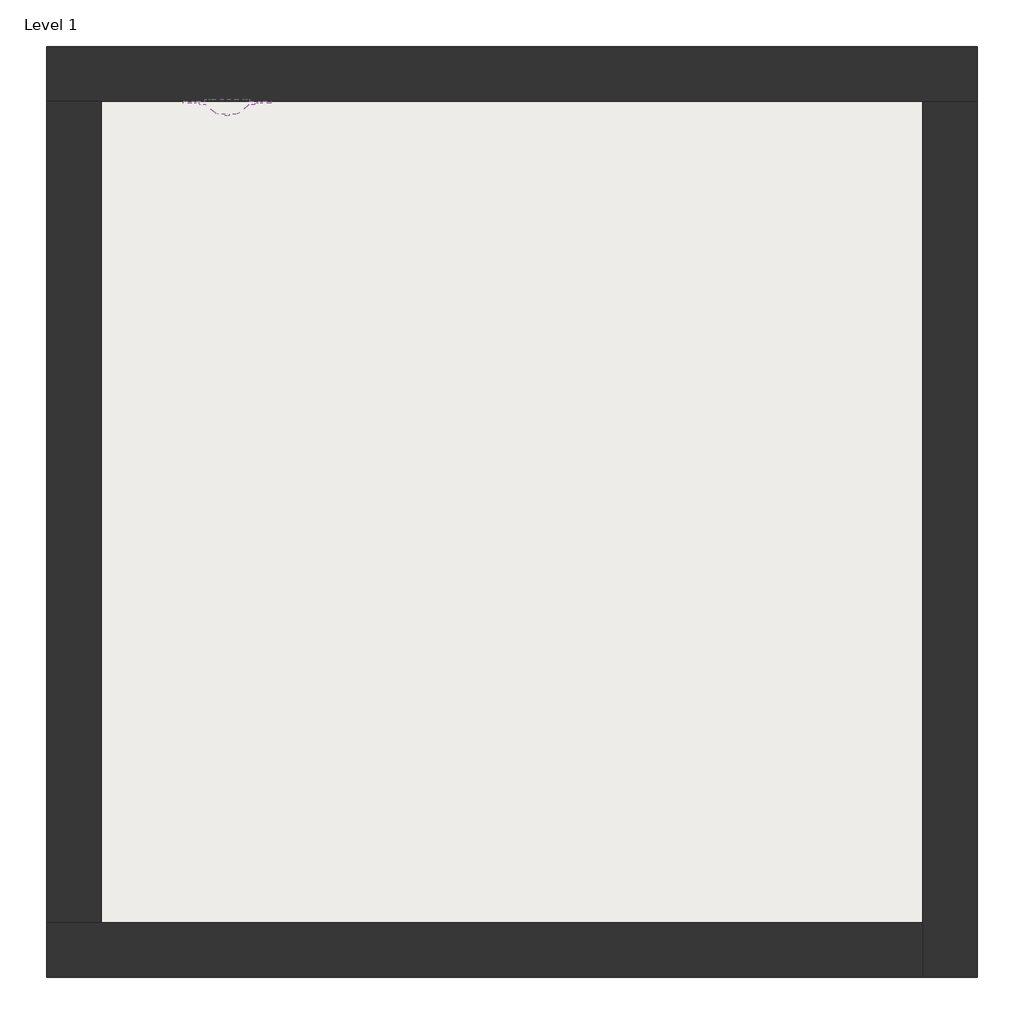
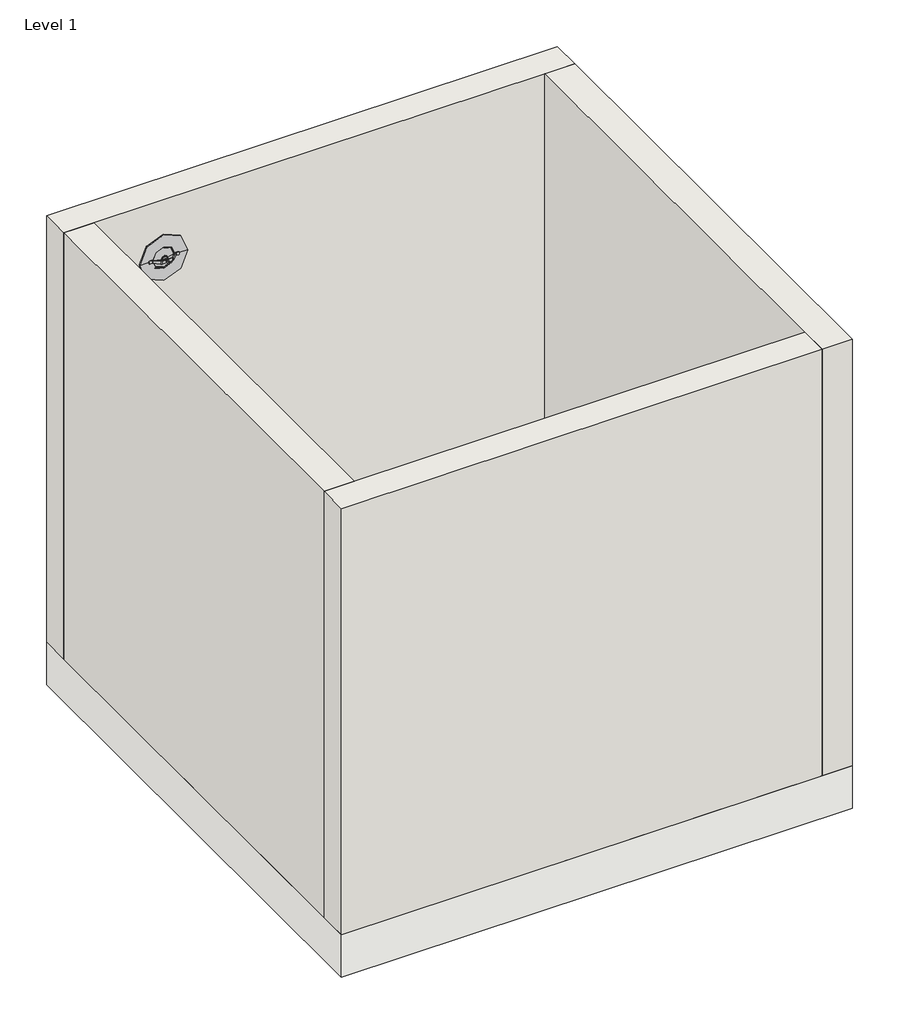
# One storey: 4 walls, 1 proxy, 1 slab.
"""IFC4 building model written with IfcOpenShell, lengths in millimetres."""

import ifcopenshell
import ifcopenshell.guid

model = None  # the IFC model being written
_history = None  # IfcOwnerHistory: only IFC2X3 demands one
_inside = {}  # id of a spatial element -> (the spatial element, [elements in it])
_under = {}  # id of a project, library or spatial element -> (it, [spatial elements below it])
_declared = {}  # id of a project -> (the project, [libraries it declares])
_typed = {}  # id of a type object -> (the type object, [elements of that type])
_made_of = {}  # id of a material, layer set ... -> (it, [elements and type objects made of it])


def new_model(schema):
    """Start an empty IFC model of exactly this schema.

    Asked for "IFC4X3", IfcOpenShell would pick the latest addendum, in which some entities
    have other attributes; the version numbers below select the first issue.
    IFC2X3 requires an IfcOwnerHistory on every rooted entity: one is made here for all.
    """
    global model, _history
    if schema == "IFC4X3":
        model = ifcopenshell.file(schema_version=(4, 3, 0, 0))
    else:
        model = ifcopenshell.file(schema=schema)
    _inside.clear()
    _under.clear()
    _declared.clear()
    _typed.clear()
    _made_of.clear()
    _history = None
    if model.schema == "IFC2X3":
        org = make("IfcOrganization", Name="unknown")
        user = make(
            "IfcPersonAndOrganization",
            ThePerson=make("IfcPerson", FamilyName="unknown"),
            TheOrganization=org,
        )
        app = make(
            "IfcApplication",
            ApplicationDeveloper=org,
            Version="unknown",
            ApplicationFullName="unknown",
            ApplicationIdentifier="unknown",
        )
        _history = make(
            "IfcOwnerHistory",
            OwningUser=user,
            OwningApplication=app,
            ChangeAction="ADDED",
            CreationDate=0,
        )
    return model


def make(cls, **values):
    """One entity of the class cls with the attributes given. An attribute that is None is left unset."""
    return model.create_entity(
        cls, **{name: value for name, value in values.items() if value is not None}
    )


def rooted(cls, **values):
    """An entity with a GlobalId (a new one), such as an element, a storey or a relation."""
    return make(cls, GlobalId=ifcopenshell.guid.new(), OwnerHistory=_history, **values)


def si_unit(unit_type, name, prefix=None):
    """IfcSIUnit, for example si_unit("LENGTHUNIT", "METRE", prefix="MILLI")."""
    return make("IfcSIUnit", UnitType=unit_type, Prefix=prefix, Name=name)


def assignment(units):
    """IfcUnitAssignment: the units of a project."""
    return None if units is None else make("IfcUnitAssignment", Units=units)


def point(xyz):
    """IfcCartesianPoint."""
    return None if xyz is None else make("IfcCartesianPoint", Coordinates=xyz)


def direction(xyz):
    """IfcDirection."""
    return None if xyz is None else make("IfcDirection", DirectionRatios=xyz)


def frame(location, z_axis=None, x_axis=None):
    """IfcAxis2Placement3D, a coordinate frame: its origin and axes. An axis left out is left unset."""
    return make(
        "IfcAxis2Placement3D",
        Location=point(location),
        Axis=direction(z_axis),
        RefDirection=direction(x_axis),
    )


def origin():
    """The frame at (0, 0, 0) with its axes left unset."""
    return frame((0.0, 0.0, 0.0))


def origin_with_axes():
    """The frame at (0, 0, 0) with the z axis (0, 0, 1) and the x axis (1, 0, 0) written out."""
    return frame((0.0, 0.0, 0.0), z_axis=(0.0, 0.0, 1.0), x_axis=(1.0, 0.0, 0.0))


def place(relative_to, where):
    """IfcLocalPlacement: puts the frame where relative to a parent placement (None: the world)."""
    return make(
        "IfcLocalPlacement", PlacementRelTo=relative_to, RelativePlacement=where
    )


def context(
    kind, dimensions, precision=None, world=None, true_north=None, identifier=None
):
    """IfcGeometricRepresentationContext, for example the 3D "Model" context."""
    return make(
        "IfcGeometricRepresentationContext",
        ContextIdentifier=identifier,
        ContextType=kind,
        CoordinateSpaceDimension=dimensions,
        Precision=precision,
        WorldCoordinateSystem=world,
        TrueNorth=true_north,
    )


def project(units=None, contexts=None):
    """IfcProject with its units and contexts."""
    return rooted(
        "IfcProject",
        Name="project",
        RepresentationContexts=contexts,
        UnitsInContext=assignment(units),
    )


def spatial(cls, under=None, at=None, **own):
    """A site, building, storey or space (cls), placed at a placement, below another one or the project."""
    s = rooted(cls, ObjectPlacement=at, **own)
    if under is not None:
        _under.setdefault(under.id(), (under, []))[1].append(s)
    return s


def polyline(points):
    """IfcPolyline through the points."""
    return make("IfcPolyline", Points=[point(p) for p in points])


def circle_curve(where, radius):
    """IfcCircle in the frame where."""
    return make("IfcCircle", Position=where, Radius=radius)


def ellipse_curve(where, semi_axis1, semi_axis2):
    """IfcEllipse in the frame where."""
    return make(
        "IfcEllipse", Position=where, SemiAxis1=semi_axis1, SemiAxis2=semi_axis2
    )


def trimmed(basis, trim1, trim2, sense, master):
    """IfcTrimmedCurve: the piece of a basis curve between two trims."""
    return make(
        "IfcTrimmedCurve",
        BasisCurve=basis,
        Trim1=trim1,
        Trim2=trim2,
        SenseAgreement=sense,
        MasterRepresentation=master,
    )


def outline(outer, holes=None, kind="AREA"):
    """IfcArbitraryClosedProfileDef: a profile drawn as a closed curve; with holes, ...WithVoids."""
    if holes is None:
        return make("IfcArbitraryClosedProfileDef", ProfileType=kind, OuterCurve=outer)
    return make(
        "IfcArbitraryProfileDefWithVoids",
        ProfileType=kind,
        OuterCurve=outer,
        InnerCurves=holes,
    )


def extrude(swept, where, along, depth):
    """IfcExtrudedAreaSolid: the profile swept, set in the frame where, extruded along a direction by depth."""
    return make(
        "IfcExtrudedAreaSolid",
        SweptArea=swept,
        Position=where,
        ExtrudedDirection=direction(along),
        Depth=depth,
    )


def faces_of(points, faces, orient=None, outer=None):
    """IfcFace entities. A face is a list of loops; a loop is a list of indices into points, from 0.

    orient and outer hold one flag for each loop. By default every Orientation is true, the
    first loop of a face is its IfcFaceOuterBound and the others are IfcFaceBound.
    """
    made = []
    for i, loops in enumerate(faces):
        bounds = []
        for j, loop in enumerate(loops):
            is_outer = j == 0 if outer is None else outer[i][j]
            bounds.append(
                make(
                    "IfcFaceOuterBound" if is_outer else "IfcFaceBound",
                    Bound=make("IfcPolyLoop", Polygon=[points[k] for k in loop]),
                    Orientation=True if orient is None else orient[i][j],
                )
            )
        made.append(make("IfcFace", Bounds=bounds))
    return made


def faceted_brep(points, faces, orient=None, outer=None, voids=None):
    """IfcFacetedBrep: a solid bounded by flat faces; with voids (closed shells), ...WithVoids."""
    shared = [point(p) for p in points]
    hull = make("IfcClosedShell", CfsFaces=faces_of(shared, faces, orient, outer))
    if voids is None:
        return make("IfcFacetedBrep", Outer=hull)
    return make(
        "IfcFacetedBrepWithVoids",
        Outer=hull,
        Voids=[
            make(cls, CfsFaces=faces_of(shared, fs, o, b)) for cls, fs, o, b in voids
        ],
    )


def shape(context_of_items, identifier, shape_type, items):
    """IfcShapeRepresentation: the items that make up one representation, for example the "Body"."""
    return make(
        "IfcShapeRepresentation",
        ContextOfItems=context_of_items,
        RepresentationIdentifier=identifier,
        RepresentationType=shape_type,
        Items=items,
    )


def source(mapping_origin, context_of_items, identifier, shape_type, items):
    """IfcRepresentationMap: a shape defined once, which mapped items show again and again."""
    return make(
        "IfcRepresentationMap",
        MappingOrigin=mapping_origin,
        MappedRepresentation=shape(context_of_items, identifier, shape_type, items),
    )


def transform(
    local_origin,
    x_axis=None,
    y_axis=None,
    z_axis=None,
    scale=None,
    scale2=None,
    scale3=None,
    uniform=True,
):
    """IfcCartesianTransformationOperator3D, or its non-uniform kind. x_axis, y_axis, z_axis: its Axis1, 2, 3."""
    if uniform:
        return make(
            "IfcCartesianTransformationOperator3D",
            Axis1=direction(x_axis),
            Axis2=direction(y_axis),
            LocalOrigin=point(local_origin),
            Scale=scale,
            Axis3=direction(z_axis),
        )
    return make(
        "IfcCartesianTransformationOperator3DnonUniform",
        Axis1=direction(x_axis),
        Axis2=direction(y_axis),
        LocalOrigin=point(local_origin),
        Scale=scale,
        Axis3=direction(z_axis),
        Scale2=scale2,
        Scale3=scale3,
    )


def mapped(mapping_source, mapping_target):
    """IfcMappedItem: shows the shape of a source again, moved by a transform."""
    return make(
        "IfcMappedItem", MappingSource=mapping_source, MappingTarget=mapping_target
    )


def made_of(thing, what):
    """Note that an element or type object is made of a material, layer set ...; save() writes the relation."""
    if what is not None:
        _made_of.setdefault(what.id(), (what, []))[1].append(thing)
    return thing


def element(
    cls,
    number,
    at=None,
    inside=None,
    cuts=None,
    type_object=None,
    material=None,
    context=None,
    identifier="Body",
    shape_type=None,
    held_by="IfcProductDefinitionShape",
    body=None,
    shapes=None,
    **own,
):
    """One element of the class cls, such as IfcWall. Its Tag is "e" and its number.

    at: its placement. inside: the storey or other place that contains it. cuts: it is an
    opening in that element (IfcRelVoidsElement). A single representation is given by context,
    identifier, shape_type and body (its items); several are given by shapes. held_by: the class
    of the entity that holds the representations. save() writes the other relations.
    """
    e = rooted(cls, Tag="e%d" % number, ObjectPlacement=at, **own)
    if body is not None:
        shapes = [shape(context, identifier, shape_type, body)]
    if shapes is not None:
        e.Representation = make(held_by, Representations=shapes)
    if inside is not None:
        _inside.setdefault(inside.id(), (inside, []))[1].append(e)
    if cuts is not None:
        rooted(
            "IfcRelVoidsElement", RelatingBuildingElement=cuts, RelatedOpeningElement=e
        )
    if type_object is not None:
        _typed.setdefault(type_object.id(), (type_object, []))[1].append(e)
    return made_of(e, material)


def aggregate(whole, parts):
    """IfcRelAggregates: a whole, such as a stair, and the parts it consists of."""
    return rooted("IfcRelAggregates", RelatingObject=whole, RelatedObjects=parts)


def save(model, path):
    """Write the relations noted so far, then the file.

    IfcRelAggregates (storeys below a building ...), IfcRelContainedInSpatialStructure (elements
    in a storey), IfcRelDefinesByType, IfcRelAssociatesMaterial and IfcRelDeclares: one each for
    every whole, place, type object, material and project.
    """
    for whole, parts in _under.values():
        aggregate(whole, parts)
    for where, things in _inside.values():
        rooted(
            "IfcRelContainedInSpatialStructure",
            RelatedElements=things,
            RelatingStructure=where,
        )
    for kind, things in _typed.values():
        rooted("IfcRelDefinesByType", RelatedObjects=things, RelatingType=kind)
    for what, things in _made_of.values():
        rooted("IfcRelAssociatesMaterial", RelatedObjects=things, RelatingMaterial=what)
    for by, libraries in _declared.values():
        rooted("IfcRelDeclares", RelatingContext=by, RelatedDefinitions=libraries)
    model.write(path)


def plane_surface(at):
    """IfcPlane: the flat surface through the origin of the frame at, square to its z axis."""
    return make("IfcPlane", Position=at)


def cylinder_surface(at, radius):
    """IfcCylindricalSurface: all points at the distance radius from the z axis of the frame at."""
    return make("IfcCylindricalSurface", Position=at, Radius=radius)


def revolved_surface(curve, axis_point, axis_direction):
    """IfcSurfaceOfRevolution: the curve turned about the line through axis_point along axis_direction."""
    return make(
        "IfcSurfaceOfRevolution",
        SweptCurve=make("IfcArbitraryOpenProfileDef", ProfileType="CURVE", Curve=curve),
        AxisPosition=make("IfcAxis1Placement", Location=point(axis_point), Axis=direction(axis_direction)),
    )


def advanced_brep(points, edges, surfaces, faces):
    """IfcAdvancedBrep: a solid bounded by faces that lie on surfaces and meet in shared edges.

    An edge is (start, end): straight between two places in points (the first is 0);
    or (start, end, curve); or (start, end, curve, False) where it runs against its curve.
    A face is (place in surfaces, loops), or (place, loops, False) where it looks against
    its surface's normal. A loop lists edges by number (the first is 1), with a minus sign
    where the edge is run from its end to its start. The first loop is the outer one.
    """
    corners = [point(p) for p in points]
    vertices = [make("IfcVertexPoint", VertexGeometry=c) for c in corners]
    made = []
    for start, end, *more in edges:
        made.append(
            make(
                "IfcEdgeCurve",
                EdgeStart=vertices[start],
                EdgeEnd=vertices[end],
                EdgeGeometry=more[0] if more else make("IfcPolyline", Points=[corners[start], corners[end]]),
                SameSense=more[1] if len(more) > 1 else True,
            )
        )
    hull = []
    for where, loops, *sense in faces:
        bounds = []
        for j, loop in enumerate(loops):
            ring = [make("IfcOrientedEdge", EdgeElement=made[abs(k) - 1], Orientation=k > 0) for k in loop]
            bounds.append(
                make(
                    "IfcFaceOuterBound" if j == 0 else "IfcFaceBound",
                    Bound=make("IfcEdgeLoop", EdgeList=ring),
                    Orientation=True,
                )
            )
        hull.append(make("IfcAdvancedFace", Bounds=bounds, FaceSurface=surfaces[where], SameSense=sense[0] if sense else True))
    return make("IfcAdvancedBrep", Outer=make("IfcClosedShell", CfsFaces=hull))


def mechanical_equipment_492a67d3(model_context):
    return source(origin(), model_context, "Body", "AdvancedBrep", [
        advanced_brep(
        [(44.3795006, 108.0, 2610.0), (54.2298211, 113.0, 2610.0), (87.44309, 140.8692417, 2610.0), (91.8102497, 143.0, 2610.0), (125.0, 143.0, 2610.0), (158.1897503, 143.0, 2610.0), (162.55691, 140.8692417, 2610.0), (195.7701789, 113.0, 2610.0), (205.6204994, 108.0, 2610.0), (221.2200072, 108.0, 2610.0), (221.2200072, 113.0, 2610.0), (205.6204994, 113.0, 2610.0), (201.5540671, 114.8851429, 2610.0), (165.874925, 144.8234979, 2610.0), (158.1897503, 148.0, 2610.0), (125.0, 148.0, 2610.0), (91.8102497, 148.0, 2610.0), (84.125075, 144.8234979, 2610.0), (48.4459329, 114.8851429, 2610.0), (44.3795006, 113.0, 2610.0), (28.7799928, 113.0, 2610.0), (28.7799928, 108.0, 2610.0), (44.3795006, 113.0, 2590.0), (48.4459329, 114.8851429, 2590.0), (84.125075, 144.8234979, 2590.0), (91.8102497, 148.0, 2590.0), (125.0, 148.0, 2590.0), (158.1897503, 148.0, 2590.0), (165.874925, 144.8234979, 2590.0), (201.5540671, 114.8851429, 2590.0), (205.6204994, 113.0, 2590.0), (221.2200072, 113.0, 2590.0), (221.2200072, 108.0, 2590.0), (205.6204994, 108.0, 2590.0), (195.7701789, 113.0, 2590.0), (162.55691, 140.8692417, 2590.0), (158.1897503, 143.0, 2590.0), (125.0, 143.0, 2590.0), (91.8102497, 143.0, 2590.0), (87.44309, 140.8692417, 2590.0), (54.2298211, 113.0, 2590.0), (44.3795006, 108.0, 2590.0), (28.7799928, 108.0, 2590.0), (28.7799928, 113.0, 2590.0), (25.0, 108.0, 2606.2200072), (25.0, 108.0, 2593.7799928), (225.0, 108.0, 2593.7799928), (225.0, 108.0, 2606.2200072), (225.0, 113.0, 2593.7799928), (225.0, 113.0, 2606.2200072), (25.0, 113.0, 2593.7799928), (25.0, 113.0, 2606.2200072)],
        [
            (0, 1, circle_curve(frame((38.5511411, 131.6851233, 2610.0), z_axis=(0.0, 0.0, 1.0), x_axis=(1.0, 0.0, 0.0)), 24.3916961)),
            (1, 2),
            (2, 3, circle_curve(frame((93.9022065, 133.1715663, 2610.0), z_axis=(0.0, 0.0, -1.0), x_axis=(1.0, 0.0, 0.0)), 10.0486015)),
            (3, 4),
            (4, 5),
            (5, 6, circle_curve(frame((156.0977935, 133.1715663, 2610.0), z_axis=(0.0, 0.0, -1.0), x_axis=(-1.0, 0.0, 0.0)), 10.0486015)),
            (6, 7),
            (7, 8, circle_curve(frame((211.4488589, 131.6851233, 2610.0), z_axis=(0.0, 0.0, 1.0), x_axis=(-1.0, 0.0, 0.0)), 24.3916961)),
            (8, 9),
            (9, 10),
            (10, 11),
            (11, 12, circle_curve(frame((205.6204994, 118.3284116, 2610.0), z_axis=(0.0, 0.0, -1.0), x_axis=(-1.0, 0.0, 0.0)), 5.3284116)),
            (12, 13),
            (13, 14, circle_curve(frame((158.1897503, 137.115059, 2610.0), z_axis=(0.0, 0.0, 1.0), x_axis=(-1.0, 0.0, 0.0)), 10.884941)),
            (14, 15),
            (15, 16),
            (16, 17, circle_curve(frame((91.8102497, 137.115059, 2610.0), z_axis=(0.0, 0.0, 1.0), x_axis=(1.0, 0.0, 0.0)), 10.884941)),
            (17, 18),
            (18, 19, circle_curve(frame((44.3795006, 118.3284116, 2610.0), z_axis=(0.0, 0.0, -1.0), x_axis=(1.0, 0.0, 0.0)), 5.3284116)),
            (19, 20),
            (20, 21),
            (21, 0),
            (22, 23, circle_curve(frame((44.3795006, 118.3284116, 2590.0), z_axis=(0.0, 0.0, 1.0), x_axis=(1.0, 0.0, 0.0)), 5.3284116)),
            (23, 24),
            (24, 25, circle_curve(frame((91.8102497, 137.115059, 2590.0), z_axis=(0.0, 0.0, -1.0), x_axis=(1.0, 0.0, 0.0)), 10.884941)),
            (25, 26),
            (26, 27),
            (27, 28, circle_curve(frame((158.1897503, 137.115059, 2590.0), z_axis=(0.0, 0.0, -1.0), x_axis=(-1.0, 0.0, 0.0)), 10.884941)),
            (28, 29),
            (29, 30, circle_curve(frame((205.6204994, 118.3284116, 2590.0), z_axis=(0.0, 0.0, 1.0), x_axis=(-1.0, 0.0, 0.0)), 5.3284116)),
            (30, 31),
            (31, 32),
            (32, 33),
            (33, 34, circle_curve(frame((211.4488589, 131.6851233, 2590.0), z_axis=(0.0, 0.0, -1.0), x_axis=(-1.0, 0.0, 0.0)), 24.3916961)),
            (34, 35),
            (35, 36, circle_curve(frame((156.0977935, 133.1715663, 2590.0), z_axis=(0.0, 0.0, 1.0), x_axis=(-1.0, 0.0, 0.0)), 10.0486015)),
            (36, 37),
            (37, 38),
            (38, 39, circle_curve(frame((93.9022065, 133.1715663, 2590.0), z_axis=(0.0, 0.0, 1.0), x_axis=(1.0, 0.0, 0.0)), 10.0486015)),
            (39, 40),
            (40, 41, circle_curve(frame((38.5511411, 131.6851233, 2590.0), z_axis=(0.0, 0.0, -1.0), x_axis=(1.0, 0.0, 0.0)), 24.3916961)),
            (41, 42),
            (42, 43),
            (43, 22),
            (41, 0),
            (21, 44, circle_curve(frame((28.7799928, 108.0, 2606.2200072), z_axis=(0.0, -1.0, 0.0), x_axis=(1.0, 0.0, 0.0)), 3.7799928)),
            (44, 45),
            (45, 42, circle_curve(frame((28.7799928, 108.0, 2593.7799928), z_axis=(0.0, -1.0, 0.0), x_axis=(1.0, 0.0, 0.0)), 3.7799928)),
            (40, 1),
            (39, 2),
            (38, 3),
            (37, 4),
            (36, 5),
            (35, 6),
            (34, 7),
            (33, 8),
            (32, 46, circle_curve(frame((221.2200072, 108.0, 2593.7799928), z_axis=(0.0, -1.0, 0.0), x_axis=(-1.0, 0.0, 0.0)), 3.7799928)),
            (46, 47),
            (47, 9, circle_curve(frame((221.2200072, 108.0, 2606.2200072), z_axis=(0.0, -1.0, 0.0), x_axis=(-1.0, 0.0, 0.0)), 3.7799928)),
            (46, 48),
            (48, 49),
            (49, 47),
            (30, 11),
            (10, 49, circle_curve(frame((221.2200072, 113.0, 2606.2200072), z_axis=(0.0, 1.0, 0.0), x_axis=(-1.0, 0.0, 0.0)), 3.7799928)),
            (48, 31, circle_curve(frame((221.2200072, 113.0, 2593.7799928), z_axis=(0.0, 1.0, 0.0), x_axis=(-1.0, 0.0, 0.0)), 3.7799928)),
            (29, 12),
            (28, 13),
            (27, 14),
            (26, 15),
            (25, 16),
            (24, 17),
            (23, 18),
            (22, 19),
            (43, 50, circle_curve(frame((28.7799928, 113.0, 2593.7799928), z_axis=(0.0, 1.0, 0.0), x_axis=(1.0, 0.0, 0.0)), 3.7799928)),
            (50, 51),
            (51, 20, circle_curve(frame((28.7799928, 113.0, 2606.2200072), z_axis=(0.0, 1.0, 0.0), x_axis=(1.0, 0.0, 0.0)), 3.7799928)),
            (44, 51),
            (50, 45),
        ],
        [
            plane_surface(frame((25.0, 108.0, 2610.0), z_axis=(0.0, 0.0, 1.0), x_axis=(1.0, 0.0, 0.0))),
            plane_surface(frame((25.0, 108.0, 2590.0), z_axis=(0.0, 0.0, -1.0), x_axis=(-1.0, 0.0, 0.0))),
            plane_surface(frame((25.0, 108.0, 2610.0), z_axis=(0.0, -1.0, 0.0), x_axis=(0.0, 0.0, -1.0))),
            cylinder_surface(frame((38.5511411, 131.6851233, 2590.0), z_axis=(0.0, 0.0, 1.0), x_axis=(1.0, 0.0, 0.0)), 24.3916961),
            plane_surface(frame((54.2298211, 113.0, 2610.0), z_axis=(0.6427876096865391, -0.7660444431189783, 0.0), x_axis=(0.0, 0.0, -1.0))),
            revolved_surface(polyline([(103.95080800000001, 133.1715663, 2590.0), (103.95080800000001, 133.1715663, 2610.0)]), (93.9022065, 133.1715663, 2590.0), (0.0, 0.0, -1.0)),
            plane_surface(frame((91.8102497, 143.0, 2610.0), z_axis=(0.0, -1.0, 0.0), x_axis=(0.0, 0.0, -1.0))),
            plane_surface(frame((125.0, 143.0, 2610.0), z_axis=(0.0, -1.0, 0.0), x_axis=(0.0, 0.0, -1.0))),
            revolved_surface(polyline([(146.049192, 133.1715663, 2590.0), (146.049192, 133.1715663, 2610.0)]), (156.0977935, 133.1715663, 2590.0), (0.0, 0.0, -1.0)),
            plane_surface(frame((162.55691, 140.8692417, 2610.0), z_axis=(-0.6427876096865387, -0.7660444431189786, 0.0), x_axis=(0.0, 0.0, -1.0))),
            cylinder_surface(frame((211.4488589, 131.6851233, 2590.0), z_axis=(0.0, 0.0, 1.0), x_axis=(-1.0, 0.0, 0.0)), 24.3916961),
            plane_surface(frame((205.6204994, 108.0, 2610.0), z_axis=(0.0, -1.0, 0.0), x_axis=(0.0, 0.0, -1.0))),
            plane_surface(frame((225.0, 108.0, 2610.0), z_axis=(1.0, 0.0, 0.0), x_axis=(0.0, 0.0, -1.0))),
            plane_surface(frame((225.0, 113.0, 2610.0), z_axis=(0.0, 1.0, 0.0), x_axis=(0.0, 0.0, -1.0))),
            revolved_surface(polyline([(200.2920878, 118.3284116, 2590.0), (200.2920878, 118.3284116, 2610.0)]), (205.6204994, 118.3284116, 2590.0), (0.0, 0.0, -1.0)),
            plane_surface(frame((201.5540671, 114.8851429, 2610.0), z_axis=(0.6427876096865414, 0.7660444431189763, 0.0), x_axis=(0.0, 0.0, -1.0))),
            cylinder_surface(frame((158.1897503, 137.115059, 2590.0), z_axis=(0.0, 0.0, 1.0), x_axis=(-1.0, 0.0, 0.0)), 10.884941),
            plane_surface(frame((158.1897503, 148.0, 2610.0), z_axis=(0.0, 1.0, 0.0), x_axis=(0.0, 0.0, -1.0))),
            plane_surface(frame((125.0, 148.0, 2610.0), z_axis=(0.0, 1.0, 0.0), x_axis=(0.0, 0.0, -1.0))),
            cylinder_surface(frame((91.8102497, 137.115059, 2590.0), z_axis=(0.0, 0.0, 1.0), x_axis=(1.0, 0.0, 0.0)), 10.884941),
            plane_surface(frame((84.125075, 144.8234979, 2610.0), z_axis=(-0.6427876096865359, 0.766044443118981, 0.0), x_axis=(0.0, 0.0, -1.0))),
            revolved_surface(polyline([(49.7079122, 118.3284116, 2590.0), (49.7079122, 118.3284116, 2610.0)]), (44.3795006, 118.3284116, 2590.0), (0.0, 0.0, -1.0)),
            plane_surface(frame((44.3795006, 113.0, 2610.0), z_axis=(0.0, 1.0, 0.0), x_axis=(0.0, 0.0, -1.0))),
            plane_surface(frame((25.0, 113.0, 2610.0), z_axis=(-1.0, 0.0, 0.0), x_axis=(0.0, 0.0, -1.0))),
            cylinder_surface(frame((28.7799928, 108.0, 2593.7799928), z_axis=(0.0, -1.0, 0.0), x_axis=(1.0, 0.0, 0.0)), 3.7799928),
            cylinder_surface(frame((28.7799928, 93.5, 2606.2200072), z_axis=(0.0, -1.0, 0.0), x_axis=(1.0, 0.0, 0.0)), 3.7799928),
            cylinder_surface(frame((221.2200072, 93.5, 2593.7799928), z_axis=(0.0, -1.0, 0.0), x_axis=(-1.0, 0.0, 0.0)), 3.7799928),
            cylinder_surface(frame((221.2200072, 93.5, 2606.2200072), z_axis=(0.0, -1.0, 0.0), x_axis=(-1.0, 0.0, 0.0)), 3.7799928),
        ],
        [
            (0, [[1, 2, 3, 4, 5, 6, 7, 8, 9, 10, 11, 12, 13, 14, 15, 16, 17, 18, 19, 20, 21, 22]]),
            (1, [[23, 24, 25, 26, 27, 28, 29, 30, 31, 32, 33, 34, 35, 36, 37, 38, 39, 40, 41, 42, 43, 44]]),
            (2, [[45, -22, 46, 47, 48, -42]]),
            (3, [[-1, -45, -41, 49]]),
            (4, [[-2, -49, -40, 50]]),
            (5, [[-3, -50, -39, 51]]),
            (6, [[-4, -51, -38, 52]]),
            (7, [[-5, -52, -37, 53]]),
            (8, [[-6, -53, -36, 54]]),
            (9, [[-7, -54, -35, 55]]),
            (10, [[-8, -55, -34, 56]]),
            (11, [[-56, -33, 57, 58, 59, -9]]),
            (12, [[-58, 60, 61, 62]]),
            (13, [[63, -11, 64, -61, 65, -31]]),
            (14, [[-12, -63, -30, 66]]),
            (15, [[-13, -66, -29, 67]]),
            (16, [[-14, -67, -28, 68]]),
            (17, [[-15, -68, -27, 69]]),
            (18, [[-16, -69, -26, 70]]),
            (19, [[-17, -70, -25, 71]]),
            (20, [[-18, -71, -24, 72]]),
            (21, [[-19, -72, -23, 73]]),
            (22, [[-73, -44, 74, 75, 76, -20]]),
            (23, [[-47, 77, -75, 78]]),
            (24, [[-43, -48, -78, -74]]),
            (25, [[-21, -76, -77, -46]]),
            (26, [[-32, -65, -60, -57]]),
            (27, [[-10, -59, -62, -64]]),
        ],
    ),
        advanced_brep(
        [(207.7271571, 93.5, 2600.0), (42.2728429, 93.5, 2600.0), (42.2728429, 97.7728429, 2600.0), (207.7271571, 97.7728429, 2600.0), (205.9367462, 93.5, 2600.0), (44.0632538, 93.5, 2600.0), (205.9367462, 97.9071057, 2600.0), (44.0632538, 97.9071057, 2600.0), (205.3438519, 98.5, 2600.0), (44.6561481, 98.5, 2600.0), (197.7785514, 98.5, 2600.0), (52.2214486, 98.5, 2600.0), (194.5390342, 101.1233093, 2600.0), (55.4609658, 101.1233093, 2600.0), (194.110594, 101.9290881, 2600.0), (55.889406, 101.9290881, 2600.0), (143.1174907, 117.056758, 2600.0), (106.8825093, 117.056758, 2600.0), (139.9690463, 120.2052024, 2600.0), (110.0309537, 120.2052024, 2600.0), (139.3942487, 120.78, 2600.0), (110.6057513, 120.78, 2600.0), (125.0, 120.78, 2600.0), (139.6388233, 122.2731901, 2600.0), (110.3611767, 122.2731901, 2600.0), (120.9566338, 122.2731901, 2600.0), (129.0433662, 122.2731901, 2600.0), (141.5029828, 120.4090307, 2600.0), (108.4970172, 120.4090307, 2600.0), (143.1991524, 118.522856, 2600.0), (106.8008476, 118.522856, 2600.0), (145.9642188, 118.2410596, 2600.0), (104.0357812, 118.2410596, 2600.0), (194.877574, 103.206216, 2600.0), (55.122426, 103.206216, 2600.0), (196.1038029, 101.6367146, 2600.0), (53.8961971, 101.6367146, 2600.0), (198.0543634, 100.0, 2600.0), (51.9456366, 100.0, 2600.0), (200.0, 100.0, 2600.0), (50.0, 100.0, 2600.0), (200.0, 108.0, 2600.0), (50.0, 108.0, 2600.0), (285.0, 108.0, 2600.0), (-35.0, 108.0, 2600.0), (285.0, 100.0, 2600.0), (-35.0, 100.0, 2600.0), (205.5, 100.0, 2600.0), (44.5, 100.0, 2600.0), (133.0867323, 136.6576943, 2600.0), (116.9132677, 136.6576943, 2600.0), (116.9132677, 153.9, 2600.0), (133.0867323, 153.9, 2600.0), (129.0433662, 136.6576943, 2600.0), (120.9566338, 136.6576943, 2600.0), (125.0, 153.9, 2600.0)],
        [
            (0, 1, circle_curve(frame((125.0, 93.5, 2600.0), z_axis=(0.0, 1.0, 0.0), x_axis=(-1.0, 0.0, 0.0)), 82.7271571)),
            (1, 2),
            (2, 3, circle_curve(frame((125.0, 97.7728429, 2600.0), z_axis=(0.0, -1.0, 0.0), x_axis=(-1.0, 0.0, 0.0)), 82.7271571)),
            (3, 0),
            (1, 0, circle_curve(frame((125.0, 93.5, 2600.0), z_axis=(0.0, 1.0, 0.0), x_axis=(-1.0, 0.0, 0.0)), 82.7271571)),
            (3, 2, circle_curve(frame((125.0, 97.7728429, 2600.0), z_axis=(0.0, -1.0, 0.0), x_axis=(-1.0, 0.0, 0.0)), 82.7271571)),
            (0, 4),
            (4, 5, circle_curve(frame((125.0, 93.5, 2600.0), z_axis=(0.0, 1.0, 0.0), x_axis=(-1.0, 0.0, 0.0)), 80.9367462)),
            (5, 1),
            (5, 4, circle_curve(frame((125.0, 93.5, 2600.0), z_axis=(0.0, 1.0, 0.0), x_axis=(-1.0, 0.0, 0.0)), 80.9367462)),
            (4, 6),
            (6, 7, circle_curve(frame((125.0, 97.9071057, 2600.0), z_axis=(0.0, 1.0, 0.0), x_axis=(-1.0, 0.0, 0.0)), 80.9367462)),
            (7, 5),
            (7, 6, circle_curve(frame((125.0, 97.9071057, 2600.0), z_axis=(0.0, 1.0, 0.0), x_axis=(-1.0, 0.0, 0.0)), 80.9367462)),
            (6, 8, circle_curve(frame((205.3438519, 97.9071057, 2600.0), z_axis=(0.0, 0.0, 1.0), x_axis=(-1.0, 0.0, 0.0)), 0.5928943)),
            (8, 9, circle_curve(frame((125.0, 98.5, 2600.0), z_axis=(0.0, 1.0, 0.0), x_axis=(-1.0, 0.0, 0.0)), 80.3438519)),
            (9, 7, circle_curve(frame((44.6561481, 97.9071057, 2600.0), z_axis=(0.0, 0.0, 1.0), x_axis=(1.0, 0.0, 0.0)), 0.5928943)),
            (9, 8, circle_curve(frame((125.0, 98.5, 2600.0), z_axis=(0.0, 1.0, 0.0), x_axis=(-1.0, 0.0, 0.0)), 80.3438519)),
            (8, 10),
            (10, 11, circle_curve(frame((125.0, 98.5, 2600.0), z_axis=(0.0, 1.0, 0.0), x_axis=(-1.0, 0.0, 0.0)), 72.7785514)),
            (11, 9),
            (11, 10, circle_curve(frame((125.0, 98.5, 2600.0), z_axis=(0.0, 1.0, 0.0), x_axis=(-1.0, 0.0, 0.0)), 72.7785514)),
            (10, 12, circle_curve(frame((197.9467336, 102.0195777, 2600.0), z_axis=(0.0, 0.0, -1.0), x_axis=(-1.0, 0.0, 0.0)), 3.5235937)),
            (12, 13, circle_curve(frame((125.0, 101.1233093, 2600.0), z_axis=(0.0, 1.0, 0.0), x_axis=(-1.0, 0.0, 0.0)), 69.5390342)),
            (13, 11, circle_curve(frame((52.0532664, 102.0195777, 2600.0), z_axis=(0.0, 0.0, -1.0), x_axis=(1.0, 0.0, 0.0)), 3.5235937)),
            (13, 12, circle_curve(frame((125.0, 101.1233093, 2600.0), z_axis=(0.0, 1.0, 0.0), x_axis=(-1.0, 0.0, 0.0)), 69.5390342)),
            (12, 14, circle_curve(frame((193.7458269, 101.2183458, 2600.0), z_axis=(0.0, 0.0, 1.0), x_axis=(-1.0, 0.0, 0.0)), 0.7988803)),
            (14, 15, circle_curve(frame((125.0, 101.9290881, 2600.0), z_axis=(0.0, 1.0, 0.0), x_axis=(-1.0, 0.0, 0.0)), 69.110594)),
            (15, 13, circle_curve(frame((56.2541731, 101.2183458, 2600.0), z_axis=(0.0, 0.0, 1.0), x_axis=(1.0, 0.0, 0.0)), 0.7988803)),
            (15, 14, circle_curve(frame((125.0, 101.9290881, 2600.0), z_axis=(0.0, 1.0, 0.0), x_axis=(-1.0, 0.0, 0.0)), 69.110594)),
            (14, 16, circle_curve(frame((128.3688639, -26.1675298, 2600.0), z_axis=(0.0, 0.0, 1.0), x_axis=(-1.0, 0.0, 0.0)), 143.9816606)),
            (16, 17, circle_curve(frame((125.0, 117.056758, 2600.0), z_axis=(0.0, 1.0, 0.0), x_axis=(-1.0, 0.0, 0.0)), 18.1174907)),
            (17, 15, circle_curve(frame((121.6311361, -26.1675298, 2600.0), z_axis=(0.0, 0.0, 1.0), x_axis=(1.0, 0.0, 0.0)), 143.9816606)),
            (17, 16, circle_curve(frame((125.0, 117.056758, 2600.0), z_axis=(0.0, 1.0, 0.0), x_axis=(-1.0, 0.0, 0.0)), 18.1174907)),
            (16, 18, circle_curve(frame((143.1174907, 120.2052024, 2600.0), z_axis=(0.0, 0.0, -1.0), x_axis=(-1.0, 0.0, 0.0)), 3.1484444)),
            (18, 19, circle_curve(frame((125.0, 120.2052024, 2600.0), z_axis=(0.0, 1.0, 0.0), x_axis=(-1.0, 0.0, 0.0)), 14.9690463)),
            (19, 17, circle_curve(frame((106.8825093, 120.2052024, 2600.0), z_axis=(0.0, 0.0, -1.0), x_axis=(1.0, 0.0, 0.0)), 3.1484444)),
            (19, 18, circle_curve(frame((125.0, 120.2052024, 2600.0), z_axis=(0.0, 1.0, 0.0), x_axis=(-1.0, 0.0, 0.0)), 14.9690463)),
            (18, 20, circle_curve(frame((139.3942487, 120.2052024, 2600.0), z_axis=(0.0, 0.0, 1.0), x_axis=(-1.0, 0.0, 0.0)), 0.5747976)),
            (20, 21, circle_curve(frame((125.0, 120.78, 2600.0), z_axis=(0.0, 1.0, 0.0), x_axis=(-1.0, 0.0, 0.0)), 14.3942487)),
            (21, 19, circle_curve(frame((110.6057513, 120.2052024, 2600.0), z_axis=(0.0, 0.0, 1.0), x_axis=(1.0, 0.0, 0.0)), 0.5747976)),
            (21, 20, circle_curve(frame((125.0, 120.78, 2600.0), z_axis=(0.0, 1.0, 0.0), x_axis=(-1.0, 0.0, 0.0)), 14.3942487)),
            (20, 22),
            (22, 21),
            (23, 24, circle_curve(frame((125.0, 122.2731901, 2600.0), z_axis=(0.0, 1.0, 0.0), x_axis=(-1.0, 0.0, 0.0)), 14.6388233)),
            (24, 25),
            (25, 26, circle_curve(frame((125.0, 122.2731901, 2600.0), z_axis=(0.0, -1.0, 0.0), x_axis=(-1.0, 0.0, 0.0)), 4.0433662)),
            (26, 23),
            (24, 23, circle_curve(frame((125.0, 122.2731901, 2600.0), z_axis=(0.0, 1.0, 0.0), x_axis=(-1.0, 0.0, 0.0)), 14.6388233)),
            (26, 25, circle_curve(frame((125.0, 122.2731901, 2600.0), z_axis=(0.0, -1.0, 0.0), x_axis=(-1.0, 0.0, 0.0)), 4.0433662)),
            (23, 27, circle_curve(frame((139.6388233, 120.4090307, 2600.0), z_axis=(0.0, 0.0, -1.0), x_axis=(-1.0, 0.0, 0.0)), 1.8641595)),
            (27, 28, circle_curve(frame((125.0, 120.4090307, 2600.0), z_axis=(0.0, 1.0, 0.0), x_axis=(-1.0, 0.0, 0.0)), 16.5029828)),
            (28, 24, circle_curve(frame((110.3611767, 120.4090307, 2600.0), z_axis=(0.0, 0.0, -1.0), x_axis=(1.0, 0.0, 0.0)), 1.8641595)),
            (28, 27, circle_curve(frame((125.0, 120.4090307, 2600.0), z_axis=(0.0, 1.0, 0.0), x_axis=(-1.0, 0.0, 0.0)), 16.5029828)),
            (27, 29, circle_curve(frame((143.3997997, 120.4090307, 2600.0), z_axis=(0.0, 0.0, 1.0), x_axis=(-1.0, 0.0, 0.0)), 1.8968169)),
            (29, 30, circle_curve(frame((125.0, 118.522856, 2600.0), z_axis=(0.0, 1.0, 0.0), x_axis=(-1.0, 0.0, 0.0)), 18.1991524)),
            (30, 28, circle_curve(frame((106.6002003, 120.4090307, 2600.0), z_axis=(0.0, 0.0, 1.0), x_axis=(1.0, 0.0, 0.0)), 1.8968169)),
            (30, 29, circle_curve(frame((125.0, 118.522856, 2600.0), z_axis=(0.0, 1.0, 0.0), x_axis=(-1.0, 0.0, 0.0)), 18.1991524)),
            (29, 31, circle_curve(frame((176.4809645, 431.386753, 2600.0), z_axis=(0.0, 0.0, 1.0), x_axis=(-1.0, 0.0, 0.0)), 314.6291421)),
            (31, 32, circle_curve(frame((125.0, 118.2410596, 2600.0), z_axis=(0.0, 1.0, 0.0), x_axis=(-1.0, 0.0, 0.0)), 20.9642188)),
            (32, 30, circle_curve(frame((73.5190355, 431.386753, 2600.0), z_axis=(0.0, 0.0, 1.0), x_axis=(1.0, 0.0, 0.0)), 314.6291421)),
            (32, 31, circle_curve(frame((125.0, 118.2410596, 2600.0), z_axis=(0.0, 1.0, 0.0), x_axis=(-1.0, 0.0, 0.0)), 20.9642188)),
            (31, 33, circle_curve(frame((131.9555378, -14.4169888, 2600.0), z_axis=(0.0, 0.0, -1.0), x_axis=(-1.0, 0.0, 0.0)), 133.3956557)),
            (33, 34, circle_curve(frame((125.0, 103.206216, 2600.0), z_axis=(0.0, 1.0, 0.0), x_axis=(-1.0, 0.0, 0.0)), 69.877574)),
            (34, 32, circle_curve(frame((118.0444622, -14.4169888, 2600.0), z_axis=(0.0, 0.0, -1.0), x_axis=(1.0, 0.0, 0.0)), 133.3956557)),
            (34, 33, circle_curve(frame((125.0, 103.206216, 2600.0), z_axis=(0.0, 1.0, 0.0), x_axis=(-1.0, 0.0, 0.0)), 69.877574)),
            (33, 35, circle_curve(frame((194.0147871, 101.2683648, 2600.0), z_axis=(0.0, 0.0, -1.0), x_axis=(-1.0, 0.0, 0.0)), 2.1212422)),
            (35, 36, circle_curve(frame((125.0, 101.6367146, 2600.0), z_axis=(0.0, 1.0, 0.0), x_axis=(-1.0, 0.0, 0.0)), 71.1038029)),
            (36, 34, circle_curve(frame((55.9852129, 101.2683648, 2600.0), z_axis=(0.0, 0.0, -1.0), x_axis=(1.0, 0.0, 0.0)), 2.1212422)),
            (36, 35, circle_curve(frame((125.0, 101.6367146, 2600.0), z_axis=(0.0, 1.0, 0.0), x_axis=(-1.0, 0.0, 0.0)), 71.1038029)),
            (35, 37, circle_curve(frame((198.0543634, 101.9806511, 2600.0), z_axis=(0.0, 0.0, 1.0), x_axis=(-1.0, 0.0, 0.0)), 1.9806511)),
            (37, 38, circle_curve(frame((125.0, 100.0, 2600.0), z_axis=(0.0, 1.0, 0.0), x_axis=(-1.0, 0.0, 0.0)), 73.0543634)),
            (38, 36, circle_curve(frame((51.9456366, 101.9806511, 2600.0), z_axis=(0.0, 0.0, 1.0), x_axis=(1.0, 0.0, 0.0)), 1.9806511)),
            (38, 37, circle_curve(frame((125.0, 100.0, 2600.0), z_axis=(0.0, 1.0, 0.0), x_axis=(-1.0, 0.0, 0.0)), 73.0543634)),
            (37, 39),
            (39, 40, circle_curve(frame((125.0, 100.0, 2600.0), z_axis=(0.0, 1.0, 0.0), x_axis=(-1.0, 0.0, 0.0)), 75.0)),
            (40, 38),
            (40, 39, circle_curve(frame((125.0, 100.0, 2600.0), z_axis=(0.0, 1.0, 0.0), x_axis=(-1.0, 0.0, 0.0)), 75.0)),
            (39, 41),
            (41, 42, circle_curve(frame((125.0, 108.0, 2600.0), z_axis=(0.0, 1.0, 0.0), x_axis=(-1.0, 0.0, 0.0)), 75.0)),
            (42, 40),
            (42, 41, circle_curve(frame((125.0, 108.0, 2600.0), z_axis=(0.0, 1.0, 0.0), x_axis=(-1.0, 0.0, 0.0)), 75.0)),
            (41, 43),
            (43, 44, circle_curve(frame((125.0, 108.0, 2600.0), z_axis=(0.0, 1.0, 0.0), x_axis=(-1.0, 0.0, 0.0)), 160.0)),
            (44, 42),
            (44, 43, circle_curve(frame((125.0, 108.0, 2600.0), z_axis=(0.0, 1.0, 0.0), x_axis=(-1.0, 0.0, 0.0)), 160.0)),
            (43, 45),
            (45, 46, circle_curve(frame((125.0, 100.0, 2600.0), z_axis=(0.0, 1.0, 0.0), x_axis=(-1.0, 0.0, 0.0)), 160.0)),
            (46, 44),
            (46, 45, circle_curve(frame((125.0, 100.0, 2600.0), z_axis=(0.0, 1.0, 0.0), x_axis=(-1.0, 0.0, 0.0)), 160.0)),
            (45, 47),
            (47, 48, circle_curve(frame((125.0, 100.0, 2600.0), z_axis=(0.0, 1.0, 0.0), x_axis=(-1.0, 0.0, 0.0)), 80.5)),
            (48, 46),
            (48, 47, circle_curve(frame((125.0, 100.0, 2600.0), z_axis=(0.0, 1.0, 0.0), x_axis=(-1.0, 0.0, 0.0)), 80.5)),
            (2, 48, circle_curve(frame((44.5, 97.7728429, 2600.0), z_axis=(0.0, 0.0, -1.0), x_axis=(1.0, 0.0, 0.0)), 2.2271571)),
            (47, 3, circle_curve(frame((205.5, 97.7728429, 2600.0), z_axis=(0.0, 0.0, -1.0), x_axis=(-1.0, 0.0, 0.0)), 2.2271571)),
            (49, 50, circle_curve(frame((125.0, 136.6576943, 2600.0), z_axis=(0.0, 1.0, 0.0), x_axis=(-1.0, 0.0, 0.0)), 8.0867323)),
            (50, 51),
            (51, 52, circle_curve(frame((125.0, 153.9, 2600.0), z_axis=(0.0, -1.0, 0.0), x_axis=(-1.0, 0.0, 0.0)), 8.0867323)),
            (52, 49),
            (50, 49, circle_curve(frame((125.0, 136.6576943, 2600.0), z_axis=(0.0, 1.0, 0.0), x_axis=(-1.0, 0.0, 0.0)), 8.0867323)),
            (52, 51, circle_curve(frame((125.0, 153.9, 2600.0), z_axis=(0.0, -1.0, 0.0), x_axis=(-1.0, 0.0, 0.0)), 8.0867323)),
            (49, 53),
            (53, 54, circle_curve(frame((125.0, 136.6576943, 2600.0), z_axis=(0.0, 1.0, 0.0), x_axis=(-1.0, 0.0, 0.0)), 4.0433662)),
            (54, 50),
            (54, 53, circle_curve(frame((125.0, 136.6576943, 2600.0), z_axis=(0.0, 1.0, 0.0), x_axis=(-1.0, 0.0, 0.0)), 4.0433662)),
            (51, 55),
            (55, 52),
            (25, 54),
            (53, 26),
        ],
        [
            cylinder_surface(frame((125.0, 193.5, 2600.0), z_axis=(0.0, -1.0, 0.0), x_axis=(-1.0, 0.0, 0.0)), 82.7271571),
            plane_surface(frame((125.0, 93.5, 2600.0), z_axis=(0.0, -1.0, 0.0), x_axis=(-1.0, 0.0, 0.0))),
            revolved_surface(polyline([(44.0632538, 93.5, 2600.0), (44.0632538, 97.9071057, 2600.0)]), (125.0, 193.5, 2600.0), (0.0, -1.0, 0.0)),
            revolved_surface(trimmed(ellipse_curve(frame((44.6561481, 97.9071057, 2600.0), z_axis=(0.0, 0.0, -1.0), x_axis=(1.0, 0.0, 0.0)), 0.5928943, 0.5928943), [point((44.0632538, 97.9071057, 2600.0))], [point((44.6561481, 98.5, 2600.0))], True, "CARTESIAN"), (125.0, 193.5, 2600.0), (0.0, -1.0, 0.0)),
            plane_surface(frame((125.0, 98.5, 2600.0), z_axis=(0.0, -1.0, 0.0), x_axis=(-1.0, 0.0, 0.0))),
            revolved_surface(trimmed(ellipse_curve(frame((52.0532664, 102.0195777, 2600.0), z_axis=(0.0, 0.0, 1.0), x_axis=(1.0, 0.0, 0.0)), 3.5235937, 3.5235937), [point((52.2214486, 98.5, 2600.0))], [point((55.4609658, 101.1233093, 2600.0))], True, "CARTESIAN"), (125.0, 193.5, 2600.0), (0.0, -1.0, 0.0)),
            revolved_surface(trimmed(ellipse_curve(frame((56.2541731, 101.2183458, 2600.0), z_axis=(0.0, 0.0, -1.0), x_axis=(1.0, 0.0, 0.0)), 0.7988803, 0.7988803), [point((55.4609658, 101.1233093, 2600.0))], [point((55.889406, 101.9290881, 2600.0))], True, "CARTESIAN"), (125.0, 193.5, 2600.0), (0.0, -1.0, 0.0)),
            revolved_surface(trimmed(ellipse_curve(frame((121.6311361, -26.1675298, 2600.0), z_axis=(0.0, 0.0, -1.0), x_axis=(1.0, 0.0, 0.0)), 143.9816606, 143.9816606), [point((55.889406, 101.9290881, 2600.0))], [point((106.8825093, 117.056758, 2600.0))], True, "CARTESIAN"), (125.0, 193.5, 2600.0), (0.0, -1.0, 0.0)),
            revolved_surface(trimmed(ellipse_curve(frame((106.8825093, 120.2052024, 2600.0), z_axis=(0.0, 0.0, 1.0), x_axis=(1.0, 0.0, 0.0)), 3.1484444, 3.1484444), [point((106.8825093, 117.056758, 2600.0))], [point((110.0309537, 120.2052024, 2600.0))], True, "CARTESIAN"), (125.0, 193.5, 2600.0), (0.0, -1.0, 0.0)),
            revolved_surface(trimmed(ellipse_curve(frame((110.6057513, 120.2052024, 2600.0), z_axis=(0.0, 0.0, -1.0), x_axis=(1.0, 0.0, 0.0)), 0.5747976, 0.5747976), [point((110.0309537, 120.2052024, 2600.0))], [point((110.6057513, 120.78, 2600.0))], True, "CARTESIAN"), (125.0, 193.5, 2600.0), (0.0, -1.0, 0.0)),
            plane_surface(frame((125.0, 120.78, 2600.0), z_axis=(0.0, -1.0, 0.0), x_axis=(-1.0, 0.0, 0.0))),
            plane_surface(frame((125.0, 122.2731901, 2600.0), z_axis=(0.0, 1.0, 0.0), x_axis=(-1.0, 0.0, 0.0))),
            revolved_surface(trimmed(ellipse_curve(frame((110.3611767, 120.4090307, 2600.0), z_axis=(0.0, 0.0, 1.0), x_axis=(1.0, 0.0, 0.0)), 1.8641595, 1.8641595), [point((110.3611767, 122.2731901, 2600.0))], [point((108.4970172, 120.4090307, 2600.0))], True, "CARTESIAN"), (125.0, 193.5, 2600.0), (0.0, -1.0, 0.0)),
            revolved_surface(trimmed(ellipse_curve(frame((106.6002003, 120.4090307, 2600.0), z_axis=(0.0, 0.0, -1.0), x_axis=(1.0, 0.0, 0.0)), 1.8968169, 1.8968169), [point((108.4970172, 120.4090307, 2600.0))], [point((106.8008476, 118.522856, 2600.0))], True, "CARTESIAN"), (125.0, 193.5, 2600.0), (0.0, -1.0, 0.0)),
            revolved_surface(trimmed(ellipse_curve(frame((73.5190355, 431.386753, 2600.0), z_axis=(0.0, 0.0, -1.0), x_axis=(1.0, 0.0, 0.0)), 314.6291421, 314.6291421), [point((106.8008476, 118.522856, 2600.0))], [point((104.0357812, 118.2410596, 2600.0))], True, "CARTESIAN"), (125.0, 193.5, 2600.0), (0.0, -1.0, 0.0)),
            revolved_surface(trimmed(ellipse_curve(frame((118.0444622, -14.4169888, 2600.0), z_axis=(0.0, 0.0, 1.0), x_axis=(1.0, 0.0, 0.0)), 133.3956557, 133.3956557), [point((104.0357812, 118.2410596, 2600.0))], [point((55.122426, 103.206216, 2600.0))], True, "CARTESIAN"), (125.0, 193.5, 2600.0), (0.0, -1.0, 0.0)),
            revolved_surface(trimmed(ellipse_curve(frame((55.9852129, 101.2683648, 2600.0), z_axis=(0.0, 0.0, 1.0), x_axis=(1.0, 0.0, 0.0)), 2.1212422, 2.1212422), [point((55.122426, 103.206216, 2600.0))], [point((53.8961971, 101.6367146, 2600.0))], True, "CARTESIAN"), (125.0, 193.5, 2600.0), (0.0, -1.0, 0.0)),
            revolved_surface(trimmed(ellipse_curve(frame((51.9456366, 101.9806511, 2600.0), z_axis=(0.0, 0.0, -1.0), x_axis=(1.0, 0.0, 0.0)), 1.9806511, 1.9806511), [point((53.8961971, 101.6367146, 2600.0))], [point((51.9456366, 100.0, 2600.0))], True, "CARTESIAN"), (125.0, 193.5, 2600.0), (0.0, -1.0, 0.0)),
            plane_surface(frame((125.0, 100.0, 2600.0), z_axis=(0.0, 1.0, 0.0), x_axis=(-1.0, 0.0, 0.0))),
            revolved_surface(polyline([(50.0, 100.0, 2600.0), (50.0, 108.0, 2600.0)]), (125.0, 193.5, 2600.0), (0.0, -1.0, 0.0)),
            plane_surface(frame((125.0, 108.0, 2600.0), z_axis=(0.0, 1.0, 0.0), x_axis=(-1.0, 0.0, 0.0))),
            cylinder_surface(frame((125.0, 193.5, 2600.0), z_axis=(0.0, -1.0, 0.0), x_axis=(-1.0, 0.0, 0.0)), 160.0),
            plane_surface(frame((125.0, 100.0, 2600.0), z_axis=(0.0, -1.0, 0.0), x_axis=(-1.0, 0.0, 0.0))),
            revolved_surface(trimmed(ellipse_curve(frame((44.5, 97.7728429, 2600.0), z_axis=(0.0, 0.0, 1.0), x_axis=(1.0, 0.0, 0.0)), 2.2271571, 2.2271571), [point((44.5, 100.0, 2600.0))], [point((42.2728429, 97.7728429, 2600.0))], True, "CARTESIAN"), (125.0, 193.5, 2600.0), (0.0, -1.0, 0.0)),
            cylinder_surface(frame((125.0, 193.5, 2600.0), z_axis=(0.0, -1.0, 0.0), x_axis=(-1.0, 0.0, 0.0)), 8.0867323),
            plane_surface(frame((125.0, 136.6576943, 2600.0), z_axis=(0.0, -1.0, 0.0), x_axis=(-1.0, 0.0, 0.0))),
            plane_surface(frame((125.0, 153.9, 2600.0), z_axis=(0.0, 1.0, 0.0), x_axis=(-1.0, 0.0, 0.0))),
            cylinder_surface(frame((125.0, 193.5, 2600.0), z_axis=(0.0, -1.0, 0.0), x_axis=(-1.0, 0.0, 0.0)), 4.0433662),
        ],
        [
            (0, [[1, 2, 3, 4]]),
            (0, [[-2, 5, -4, 6]]),
            (1, [[-1, 7, 8, 9]]),
            (1, [[-5, -9, 10, -7]]),
            (2, [[-8, 11, 12, 13]]),
            (2, [[-10, -13, 14, -11]]),
            (3, [[-12, 15, 16, 17]]),
            (3, [[-14, -17, 18, -15]]),
            (4, [[-16, 19, 20, 21]]),
            (4, [[-18, -21, 22, -19]]),
            (5, [[-20, 23, 24, 25]]),
            (5, [[-22, -25, 26, -23]]),
            (6, [[-24, 27, 28, 29]]),
            (6, [[-26, -29, 30, -27]]),
            (7, [[-28, 31, 32, 33]]),
            (7, [[-30, -33, 34, -31]]),
            (8, [[-32, 35, 36, 37]]),
            (8, [[-34, -37, 38, -35]]),
            (9, [[-36, 39, 40, 41]]),
            (9, [[-38, -41, 42, -39]]),
            (10, [[-40, 43, 44]]),
            (10, [[-42, -44, -43]]),
            (11, [[45, 46, 47, 48]]),
            (11, [[-46, 49, -48, 50]]),
            (12, [[-45, 51, 52, 53]]),
            (12, [[-49, -53, 54, -51]]),
            (13, [[-52, 55, 56, 57]]),
            (13, [[-54, -57, 58, -55]]),
            (14, [[-56, 59, 60, 61]]),
            (14, [[-58, -61, 62, -59]]),
            (15, [[-60, 63, 64, 65]]),
            (15, [[-62, -65, 66, -63]]),
            (16, [[-64, 67, 68, 69]]),
            (16, [[-66, -69, 70, -67]]),
            (17, [[-68, 71, 72, 73]]),
            (17, [[-70, -73, 74, -71]]),
            (18, [[-72, 75, 76, 77]]),
            (18, [[-74, -77, 78, -75]]),
            (19, [[-76, 79, 80, 81]]),
            (19, [[-78, -81, 82, -79]]),
            (20, [[-80, 83, 84, 85]]),
            (20, [[-82, -85, 86, -83]]),
            (21, [[-84, 87, 88, 89]]),
            (21, [[-86, -89, 90, -87]]),
            (22, [[-88, 91, 92, 93]]),
            (22, [[-90, -93, 94, -91]]),
            (23, [[-3, 95, -92, 96]]),
            (23, [[-6, -96, -94, -95]]),
            (24, [[97, 98, 99, 100]]),
            (24, [[-98, 101, -100, 102]]),
            (25, [[-97, 103, 104, 105]]),
            (25, [[-101, -105, 106, -103]]),
            (26, [[-99, 107, 108]]),
            (26, [[-102, -108, -107]]),
            (27, [[-47, 109, -104, 110]]),
            (27, [[-50, -110, -106, -109]]),
        ],
    ),
    ])


model = new_model("IFC4")

# Units and contexts
model_context = context("Model", 3, world=origin())
ifc_project = project(units=[si_unit("LENGTHUNIT", "METRE", prefix="MILLI")], contexts=[model_context])

# Site, building, storey
site = spatial("IfcSite", under=ifc_project)
building = spatial("IfcBuilding", under=site)
storey = spatial("IfcBuildingStorey", under=building, Name="Level 1", Elevation=0.0)

# Proxy
placement = place(None, origin())
mechanical_equipment_shape = mechanical_equipment_492a67d3(model_context)
element("IfcBuildingElementProxy", 1, Name="BVNC 300 8Y. : BVNC 300 8Y", ObjectType="BVNC 300 8Y. : BVNC 300 8Y", at=placement, inside=storey, context=model_context, shape_type="MappedRepresentation", body=[
    mapped(mechanical_equipment_shape, transform((-10336.3122346, 11113.1412882, 0.0), x_axis=(-1.0, 0.0, 0.0), y_axis=(0.0, -1.0, 0.0), z_axis=(0.0, 0.0, 1.0))),
])

# Slab
element("IfcSlab", 2, ObjectType="Generic 300mm", at=placement, inside=storey, context=model_context, shape_type="SweptSolid", body=[
    extrude(outline(polyline([(-7721.3122346, 11213.1412882), (-7721.3122346, 7813.1412882), (-11121.3122346, 7813.1412882), (-11121.3122346, 11213.1412882), (-7721.3122346, 11213.1412882)])), frame((0.0, 0.0, -300.0), z_axis=(0.0, 0.0, 1.0), x_axis=(1.0, 0.0, 0.0)), (0.0, 0.0, 1.0), 300.0),
])

# Walls
element("IfcWall", 3, ObjectType="Generic - 200mm", at=placement, inside=storey, context=model_context, shape_type="Brep", body=[
    faceted_brep([(-11121.3122346, 11013.1412882, 0.0), (-10921.3122346, 11013.1412882, 0.0), (-7921.3122346, 11013.1412882, 0.0), (-7721.3122346, 11013.1412882, 0.0), (-7721.3122346, 11013.1412882, 3000.0), (-7921.3122346, 11013.1412882, 3000.0), (-10921.3122346, 11013.1412882, 3000.0), (-11121.3122346, 11013.1412882, 3000.0), (-11121.3122346, 11213.1412882, 0.0), (-11121.3122346, 11213.1412882, 3000.0), (-7721.3122346, 11213.1412882, 3000.0), (-7721.3122346, 11213.1412882, 0.0)], [[[0, 1, 2, 3, 4, 5, 6, 7]], [[8, 9, 10, 11]], [[3, 2, 1, 0, 8, 11]], [[7, 6, 5, 4, 10, 9]], [[4, 3, 11, 10]], [[0, 7, 9, 8]]]),
])
element("IfcWall", 4, ObjectType="Generic - 200mm", at=placement, inside=storey, context=model_context, shape_type="Brep", body=[
    faceted_brep([(-7921.3122346, 11013.1412882, 0.0), (-7921.3122346, 8013.1412882, 0.0), (-7921.3122346, 7813.1412882, 0.0), (-7921.3122346, 7813.1412882, 3000.0), (-7921.3122346, 8013.1412882, 3000.0), (-7921.3122346, 11013.1412882, 3000.0), (-7721.3122346, 11013.1412882, 0.0), (-7721.3122346, 11013.1412882, 3000.0), (-7721.3122346, 7813.1412882, 3000.0), (-7721.3122346, 7813.1412882, 0.0)], [[[0, 1, 2, 3, 4, 5]], [[6, 7, 8, 9]], [[2, 1, 0, 6, 9]], [[5, 4, 3, 8, 7]], [[0, 5, 7, 6]], [[3, 2, 9, 8]]]),
])
element("IfcWall", 5, ObjectType="Generic - 200mm", at=placement, inside=storey, context=model_context, shape_type="Brep", body=[
    faceted_brep([(-7921.3122346, 8013.1412882, 0.0), (-10921.3122346, 8013.1412882, 0.0), (-11121.3122346, 8013.1412882, 0.0), (-11121.3122346, 8013.1412882, 3000.0), (-10921.3122346, 8013.1412882, 3000.0), (-7921.3122346, 8013.1412882, 3000.0), (-7921.3122346, 7813.1412882, 0.0), (-7921.3122346, 7813.1412882, 3000.0), (-11121.3122346, 7813.1412882, 3000.0), (-11121.3122346, 7813.1412882, 0.0)], [[[0, 1, 2, 3, 4, 5]], [[6, 7, 8, 9]], [[2, 1, 0, 6, 9]], [[5, 4, 3, 8, 7]], [[0, 5, 7, 6]], [[3, 2, 9, 8]]]),
])
element("IfcWall", 6, ObjectType="Generic - 200mm", at=placement, inside=storey, context=model_context, shape_type="SweptSolid", body=[
    extrude(outline(polyline([(-10921.3122346, 11013.1412882), (-10921.3122346, 8013.1412882), (-11121.3122346, 8013.1412882), (-11121.3122346, 11013.1412882), (-10921.3122346, 11013.1412882)])), origin_with_axes(), (0.0, 0.0, 1.0), 3000.0),
])

save(model, "model.ifc")

# Revit data of these elements
# Project information
#   Project Issue Date = "Issue Date"
#   Project Status = "Project Status"
#   Client Name = "Owner"
#   Project Address = "Enter address here"
#   Project Name = "Project Name"
#   Project Number = "Project Number"
# Type "BVNC 300 8Y. : BVNC 300 8Y"
#   FLANGE HEIGHT [instance default] = 2600 mm
#   BVNC 3008Y = yes
#   Default Elevation = 0
# Type "Generic 300mm"
#   Function = 0
#   Layers, outside or top first: 300 mm no material (function 1)
# Type "Generic - 200mm"
#   Layers, outside or top first: 200 mm no material (function 1)
# Element 1 (IfcBuildingElementProxy, "BVNC 300 8Y. : BVNC 300 8Y")
#   Mark = "17"
#   FLANGE HEIGHT = 2600 mm
#   Phase Created = New Construction
# Element 2 (IfcSlab, "Generic 300mm")
#   Height Offset From Level = 0 mm
#   Phase Created = New Construction
#   Materials on its faces: "Default Floor"
# Elements 3, 4, 5, 6 (IfcWall, "Generic - 200mm")
#   Top Offset = 0 mm
#   Base Offset = 0 mm
#   Unconnected Height = 3000 mm
#   wall height = 3000 mm
#   Phase Created = New Construction
#   Base Constraint = Level 1
#   Materials on its faces: "Default Wall"
# Materials
#   "Default Floor": class "Miscellaneous", colour RGB 127 127 127, transparency 0, Cost = 0
#   "Default Wall": class "Miscellaneous", colour RGB 128 128 128, transparency 0, Cost = 0
